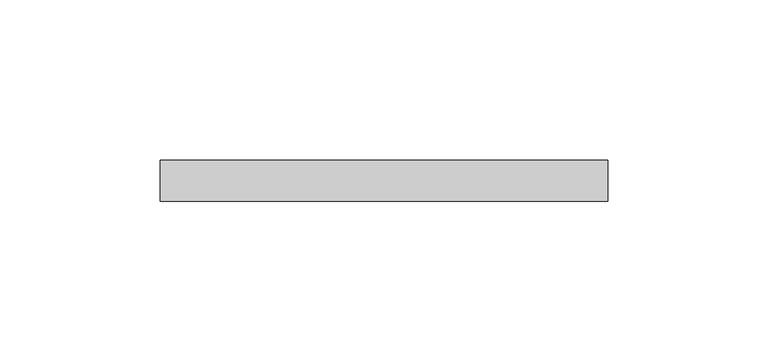
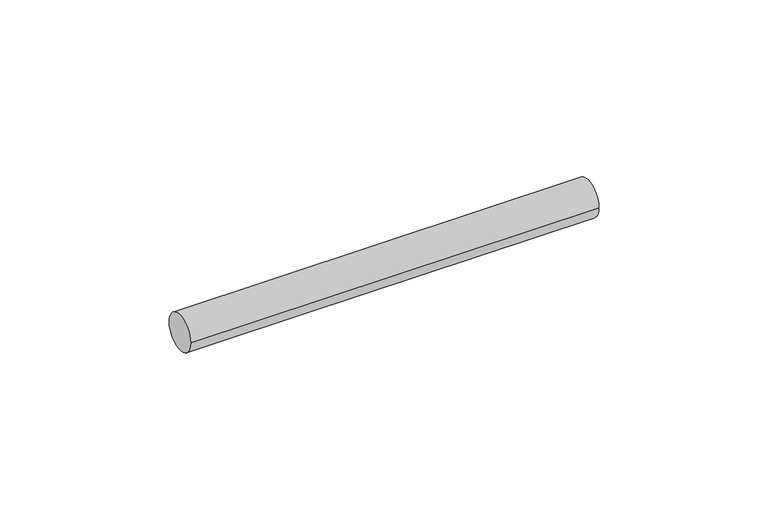
"""IFC4 building model written with IfcOpenShell, lengths in millimetres: proxy geometry, Generic Models 7:Generic Models 1:8:Generic Models 1:8 : Generic Models 7:Generic Models 1:337419:57 : Generic Models 7:Generic Models 1:8:Generic Models 1:8 : Generic Models 7:Generic Models 1:337419:315935."""

import ifcopenshell
import ifcopenshell.guid

model = None  # the IFC model being written
_history = None  # IfcOwnerHistory: only IFC2X3 demands one
_inside = {}  # id of a spatial element -> (the spatial element, [elements in it])
_under = {}  # id of a project, library or spatial element -> (it, [spatial elements below it])
_declared = {}  # id of a project -> (the project, [libraries it declares])
_typed = {}  # id of a type object -> (the type object, [elements of that type])
_made_of = {}  # id of a material, layer set ... -> (it, [elements and type objects made of it])


def new_model(schema):
    """Start an empty IFC model of exactly this schema.

    Asked for "IFC4X3", IfcOpenShell would pick the latest addendum, in which some entities
    have other attributes; the version numbers below select the first issue.
    IFC2X3 requires an IfcOwnerHistory on every rooted entity: one is made here for all.
    """
    global model, _history
    if schema == "IFC4X3":
        model = ifcopenshell.file(schema_version=(4, 3, 0, 0))
    else:
        model = ifcopenshell.file(schema=schema)
    _inside.clear()
    _under.clear()
    _declared.clear()
    _typed.clear()
    _made_of.clear()
    _history = None
    if model.schema == "IFC2X3":
        org = make("IfcOrganization", Name="unknown")
        user = make(
            "IfcPersonAndOrganization",
            ThePerson=make("IfcPerson", FamilyName="unknown"),
            TheOrganization=org,
        )
        app = make(
            "IfcApplication",
            ApplicationDeveloper=org,
            Version="unknown",
            ApplicationFullName="unknown",
            ApplicationIdentifier="unknown",
        )
        _history = make(
            "IfcOwnerHistory",
            OwningUser=user,
            OwningApplication=app,
            ChangeAction="ADDED",
            CreationDate=0,
        )
    return model


def make(cls, **values):
    """One entity of the class cls with the attributes given. An attribute that is None is left unset."""
    return model.create_entity(
        cls, **{name: value for name, value in values.items() if value is not None}
    )


def rooted(cls, **values):
    """An entity with a GlobalId (a new one), such as an element, a storey or a relation."""
    return make(cls, GlobalId=ifcopenshell.guid.new(), OwnerHistory=_history, **values)


def si_unit(unit_type, name, prefix=None):
    """IfcSIUnit, for example si_unit("LENGTHUNIT", "METRE", prefix="MILLI")."""
    return make("IfcSIUnit", UnitType=unit_type, Prefix=prefix, Name=name)


def assignment(units):
    """IfcUnitAssignment: the units of a project."""
    return None if units is None else make("IfcUnitAssignment", Units=units)


def point(xyz):
    """IfcCartesianPoint."""
    return None if xyz is None else make("IfcCartesianPoint", Coordinates=xyz)


def direction(xyz):
    """IfcDirection."""
    return None if xyz is None else make("IfcDirection", DirectionRatios=xyz)


def frame(location, z_axis=None, x_axis=None):
    """IfcAxis2Placement3D, a coordinate frame: its origin and axes. An axis left out is left unset."""
    return make(
        "IfcAxis2Placement3D",
        Location=point(location),
        Axis=direction(z_axis),
        RefDirection=direction(x_axis),
    )


def frame_2d(location, x_axis=None):
    """IfcAxis2Placement2D, a coordinate frame in the plane: its origin and x axis."""
    return make(
        "IfcAxis2Placement2D", Location=point(location), RefDirection=direction(x_axis)
    )


def origin():
    """The frame at (0, 0, 0) with its axes left unset."""
    return frame((0.0, 0.0, 0.0))


def place(relative_to, where):
    """IfcLocalPlacement: puts the frame where relative to a parent placement (None: the world)."""
    return make(
        "IfcLocalPlacement", PlacementRelTo=relative_to, RelativePlacement=where
    )


def context(
    kind, dimensions, precision=None, world=None, true_north=None, identifier=None
):
    """IfcGeometricRepresentationContext, for example the 3D "Model" context."""
    return make(
        "IfcGeometricRepresentationContext",
        ContextIdentifier=identifier,
        ContextType=kind,
        CoordinateSpaceDimension=dimensions,
        Precision=precision,
        WorldCoordinateSystem=world,
        TrueNorth=true_north,
    )


def project(units=None, contexts=None):
    """IfcProject with its units and contexts."""
    return rooted(
        "IfcProject",
        Name="project",
        RepresentationContexts=contexts,
        UnitsInContext=assignment(units),
    )


def spatial(cls, under=None, at=None, **own):
    """A site, building, storey or space (cls), placed at a placement, below another one or the project."""
    s = rooted(cls, ObjectPlacement=at, **own)
    if under is not None:
        _under.setdefault(under.id(), (under, []))[1].append(s)
    return s


def circle_curve(where, radius):
    """IfcCircle in the frame where."""
    return make("IfcCircle", Position=where, Radius=radius)


def trimmed(basis, trim1, trim2, sense, master):
    """IfcTrimmedCurve: the piece of a basis curve between two trims."""
    return make(
        "IfcTrimmedCurve",
        BasisCurve=basis,
        Trim1=trim1,
        Trim2=trim2,
        SenseAgreement=sense,
        MasterRepresentation=master,
    )


def segment(curve, same_sense, transition):
    """IfcCompositeCurveSegment."""
    return make(
        "IfcCompositeCurveSegment",
        Transition=transition,
        SameSense=same_sense,
        ParentCurve=curve,
    )


def composite_curve(segments, self_intersect=None):
    """IfcCompositeCurve: segments joined end to end."""
    return make("IfcCompositeCurve", Segments=segments, SelfIntersect=self_intersect)


def outline(outer, holes=None, kind="AREA"):
    """IfcArbitraryClosedProfileDef: a profile drawn as a closed curve; with holes, ...WithVoids."""
    if holes is None:
        return make("IfcArbitraryClosedProfileDef", ProfileType=kind, OuterCurve=outer)
    return make(
        "IfcArbitraryProfileDefWithVoids",
        ProfileType=kind,
        OuterCurve=outer,
        InnerCurves=holes,
    )


def extrude(swept, where, along, depth):
    """IfcExtrudedAreaSolid: the profile swept, set in the frame where, extruded along a direction by depth."""
    return make(
        "IfcExtrudedAreaSolid",
        SweptArea=swept,
        Position=where,
        ExtrudedDirection=direction(along),
        Depth=depth,
    )


def shape(context_of_items, identifier, shape_type, items):
    """IfcShapeRepresentation: the items that make up one representation, for example the "Body"."""
    return make(
        "IfcShapeRepresentation",
        ContextOfItems=context_of_items,
        RepresentationIdentifier=identifier,
        RepresentationType=shape_type,
        Items=items,
    )


def source(mapping_origin, context_of_items, identifier, shape_type, items):
    """IfcRepresentationMap: a shape defined once, which mapped items show again and again."""
    return make(
        "IfcRepresentationMap",
        MappingOrigin=mapping_origin,
        MappedRepresentation=shape(context_of_items, identifier, shape_type, items),
    )


def transform(
    local_origin,
    x_axis=None,
    y_axis=None,
    z_axis=None,
    scale=None,
    scale2=None,
    scale3=None,
    uniform=True,
):
    """IfcCartesianTransformationOperator3D, or its non-uniform kind. x_axis, y_axis, z_axis: its Axis1, 2, 3."""
    if uniform:
        return make(
            "IfcCartesianTransformationOperator3D",
            Axis1=direction(x_axis),
            Axis2=direction(y_axis),
            LocalOrigin=point(local_origin),
            Scale=scale,
            Axis3=direction(z_axis),
        )
    return make(
        "IfcCartesianTransformationOperator3DnonUniform",
        Axis1=direction(x_axis),
        Axis2=direction(y_axis),
        LocalOrigin=point(local_origin),
        Scale=scale,
        Axis3=direction(z_axis),
        Scale2=scale2,
        Scale3=scale3,
    )


def mapped(mapping_source, mapping_target):
    """IfcMappedItem: shows the shape of a source again, moved by a transform."""
    return make(
        "IfcMappedItem", MappingSource=mapping_source, MappingTarget=mapping_target
    )


def made_of(thing, what):
    """Note that an element or type object is made of a material, layer set ...; save() writes the relation."""
    if what is not None:
        _made_of.setdefault(what.id(), (what, []))[1].append(thing)
    return thing


def element(
    cls,
    number,
    at=None,
    inside=None,
    cuts=None,
    type_object=None,
    material=None,
    context=None,
    identifier="Body",
    shape_type=None,
    held_by="IfcProductDefinitionShape",
    body=None,
    shapes=None,
    **own,
):
    """One element of the class cls, such as IfcWall. Its Tag is "e" and its number.

    at: its placement. inside: the storey or other place that contains it. cuts: it is an
    opening in that element (IfcRelVoidsElement). A single representation is given by context,
    identifier, shape_type and body (its items); several are given by shapes. held_by: the class
    of the entity that holds the representations. save() writes the other relations.
    """
    e = rooted(cls, Tag="e%d" % number, ObjectPlacement=at, **own)
    if body is not None:
        shapes = [shape(context, identifier, shape_type, body)]
    if shapes is not None:
        e.Representation = make(held_by, Representations=shapes)
    if inside is not None:
        _inside.setdefault(inside.id(), (inside, []))[1].append(e)
    if cuts is not None:
        rooted(
            "IfcRelVoidsElement", RelatingBuildingElement=cuts, RelatedOpeningElement=e
        )
    if type_object is not None:
        _typed.setdefault(type_object.id(), (type_object, []))[1].append(e)
    return made_of(e, material)


def aggregate(whole, parts):
    """IfcRelAggregates: a whole, such as a stair, and the parts it consists of."""
    return rooted("IfcRelAggregates", RelatingObject=whole, RelatedObjects=parts)


def save(model, path):
    """Write the relations noted so far, then the file.

    IfcRelAggregates (storeys below a building ...), IfcRelContainedInSpatialStructure (elements
    in a storey), IfcRelDefinesByType, IfcRelAssociatesMaterial and IfcRelDeclares: one each for
    every whole, place, type object, material and project.
    """
    for whole, parts in _under.values():
        aggregate(whole, parts)
    for where, things in _inside.values():
        rooted(
            "IfcRelContainedInSpatialStructure",
            RelatedElements=things,
            RelatingStructure=where,
        )
    for kind, things in _typed.values():
        rooted("IfcRelDefinesByType", RelatedObjects=things, RelatingType=kind)
    for what, things in _made_of.values():
        rooted("IfcRelAssociatesMaterial", RelatedObjects=things, RelatingMaterial=what)
    for by, libraries in _declared.values():
        rooted("IfcRelDeclares", RelatingContext=by, RelatedDefinitions=libraries)
    model.write(path)


def generic_models_253af093(model_context):
    return source(origin(), model_context, "Body", "SweptSolid", [
        extrude(outline(composite_curve([segment(trimmed(circle_curve(frame_2d((-564915.9326015, 8768.3767235)), 6.35), [point((-564909.5826015, 8768.3767235))], [point((-564922.2826015, 8768.3767235))], False, "CARTESIAN"), True, "CONTINUOUS"), segment(trimmed(circle_curve(frame_2d((-564915.9326015, 8768.3767235)), 6.35), [point((-564922.2826015, 8768.3767235))], [point((-564909.5826015, 8768.3767235))], False, "CARTESIAN"), True, "CONTINUOUS")], self_intersect=False)), frame((593665.2601618, 0.0, 0.0), z_axis=(1.0, 0.0, 0.0), x_axis=(0.0, 1.0, 0.0)), (0.0, 0.0, 1.0), 139.3031242),
    ])


if __name__ == "__main__":
    model = new_model("IFC4")
    model_context = context("Model", 3, world=origin())
    ifc_project = project(units=[si_unit("LENGTHUNIT", "METRE", prefix="MILLI")], contexts=[model_context])
    site = spatial("IfcSite", under=ifc_project)
    building = spatial("IfcBuilding", under=site)
    placement = place(None, origin())
    generic_models_shape = generic_models_253af093(model_context)
    element("IfcBuildingElementProxy", 1, Name="Generic Models 7:Generic Models 1:8:Generic Models 1:8 : Generic Models 7:Generic Models 1:337419:57 : Generic Models 7:Generic Models 1:8:Generic Models 1:8 : Generic Models 7:Generic Models 1:337419:315935", ObjectType="Generic Models 7:Generic Models 1:8:Generic Models 1:8 : Generic Models 7:Generic Models 1:337419:57 : Generic Models 7:Generic Models 1:8:Generic Models 1:8 : Generic Models 7:Generic Models 1:337419:315935", at=placement, inside=building, context=model_context, shape_type="MappedRepresentation", body=[
        mapped(generic_models_shape, transform((0.0, 0.0, 0.0), x_axis=(1.0, 0.0, 0.0), y_axis=(0.0, 1.0, 0.0), z_axis=(0.0, 0.0, 1.0))),
    ])
    save(model, "model.ifc")

# Revit data of these elements
# Type "Generic Models 7:Generic Models 1:8:Generic Models 1:8 : Generic Models 7:Generic Models 1:337419:57 : Generic Models 7:Generic Models 1:8:Generic Models 1:8 : Generic Models 7:Generic Models 1:337419:315935"
#   NameOverride = "Generic Models 7:Generic Models 1:8:Generic Models 1:8 : Generic Models 7:Generic Models 1:337419:315935"
#   ObjectTypeOverride = "Generic Models 1:8 : Generic Models 7:Generic Models 1:337419"
#   Reference = "Generic Models 1"
#   Tag = "315935"
# Element 1 (IfcBuildingElementProxy, "Generic Models 7:Generic Models 1:8:Generic Models 1:8 : Generic Models 7:Generic Models 1:337419:57 : Generic Models 7:Generic Models 1:8:Generic Models 1:8 : Generic Models 7:Generic Models 1:337419:315935")
#   Materials on its faces: "0.179\" THICK BENT STEEL CLIPS"
# Materials
#   "0.179\" THICK BENT STEEL CLIPS": class "Metal", colour RGB 189 187 185, transparency 0, Description = "Structural steel 50ksi", Cost = 0
